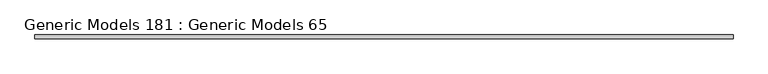
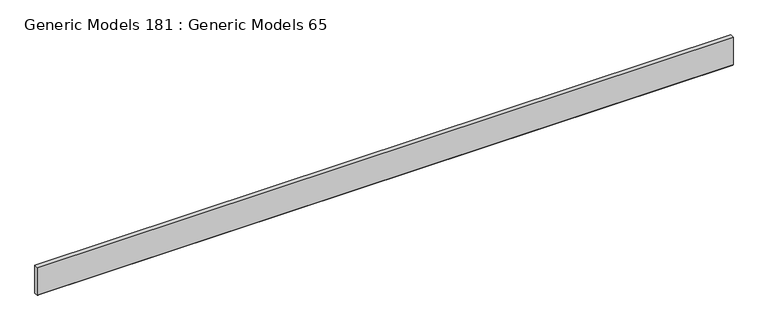
"""IFC4 building model written with IfcOpenShell, lengths in millimetres: proxy geometry, Generic Models 181 : Generic Models 65."""

from ifc_helpers import new_model, si_unit, frame, origin, place, context, project, spatial, polyline, outline, extrude, source, transform, mapped, element, save


def generic_models_181_generic_models_65_82d98486(model_context):
    return source(origin(), model_context, "Body", "SweptSolid", [
        extrude(outline(polyline([(528.6375, 508.0), (547.6875, 508.0), (547.6875, 368.3), (529.828125, 368.3), (528.6375, 369.490625), (528.6375, 508.0)])), frame((-251067.8875, 0.0, 0.0), z_axis=(1.0, 0.0, 0.0), x_axis=(0.0, 1.0, 0.0)), (0.0, 0.0, 1.0), 3289.3),
    ])


if __name__ == "__main__":
    model = new_model("IFC4")
    model_context = context("Model", 3, world=origin())
    ifc_project = project(units=[si_unit("LENGTHUNIT", "METRE", prefix="MILLI")], contexts=[model_context])
    site = spatial("IfcSite", under=ifc_project)
    building = spatial("IfcBuilding", under=site)
    placement = place(None, origin())
    generic_models_181_generic_models_65_shape = generic_models_181_generic_models_65_82d98486(model_context)
    element("IfcBuildingElementProxy", 1, Name="Generic Models 181 : Generic Models 65", ObjectType="Generic Models 181 : Generic Models 65", at=placement, inside=building, context=model_context, shape_type="MappedRepresentation", body=[
        mapped(generic_models_181_generic_models_65_shape, transform((0.0, 0.0, 0.0), x_axis=(1.0, 0.0, 0.0), y_axis=(0.0, 1.0, 0.0), z_axis=(0.0, 0.0, 1.0))),
    ])
    save(model, "model.ifc")

# Revit data of these elements
# Element 1 (IfcBuildingElementProxy, "Generic Models 181 : Generic Models 65")
#   Materials on its faces: "HORIZONTAL 1X6 CEDAR PLANKS W/ CLEAR WOOD SEALER"
# Materials
#   "HORIZONTAL 1X6 CEDAR PLANKS W/ CLEAR WOOD SEALER": class "Wood", colour RGB 234 198 147, transparency 0, Description = "Pinus Echinata", Cost = 0
